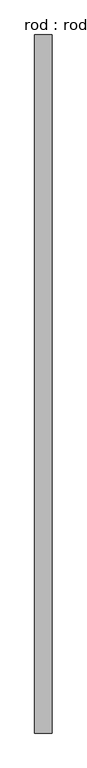
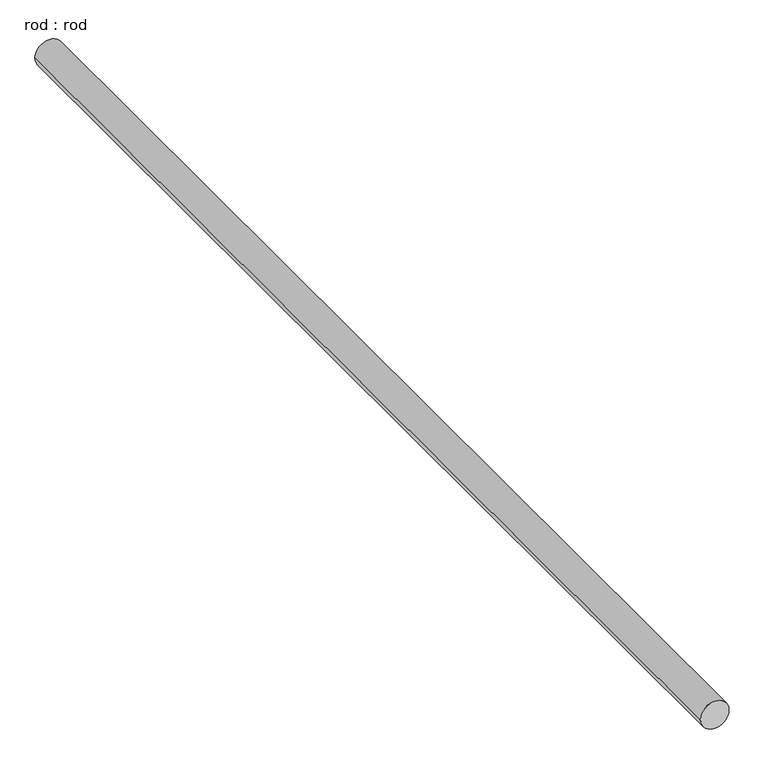
"""IFC4 building model written with IfcOpenShell, lengths in millimetres: proxy geometry, rod : rod."""

from ifc_helpers import new_model, si_unit, point, frame, frame_2d, origin, place, context, project, spatial, circle_curve, trimmed, segment, composite_curve, outline, extrude, source, transform, mapped, element, save


def rod_rod_5b3b0a5f(model_context):
    return source(origin(), model_context, "Body", "SweptSolid", [
        extrude(outline(composite_curve([segment(trimmed(circle_curve(frame_2d((0.0108462, 0.0)), 200.0), [point((0.0108462, 200.0))], [point((0.0108462, -200.0))], False, "CARTESIAN"), True, "CONTINUOUS"), segment(trimmed(circle_curve(frame_2d((0.0108462, 0.0)), 200.0), [point((0.0108462, -200.0))], [point((0.0108462, 200.0))], False, "CARTESIAN"), True, "CONTINUOUS")], self_intersect=False)), frame((0.0, -3950.3087844, 0.0), z_axis=(0.0, 1.0, 0.0), x_axis=(0.0, 0.0, 1.0)), (0.0, 0.0, 1.0), 16086.0747995),
    ])


if __name__ == "__main__":
    model = new_model("IFC4")
    model_context = context("Model", 3, world=origin())
    ifc_project = project(units=[si_unit("LENGTHUNIT", "METRE", prefix="MILLI")], contexts=[model_context])
    site = spatial("IfcSite", under=ifc_project)
    building = spatial("IfcBuilding", under=site)
    placement = place(None, origin())
    rod_rod_shape = rod_rod_5b3b0a5f(model_context)
    element("IfcBuildingElementProxy", 1, Name="rod : rod", ObjectType="rod : rod", at=placement, inside=building, context=model_context, shape_type="MappedRepresentation", body=[
        mapped(rod_rod_shape, transform((0.0, 0.0, 0.0), x_axis=(1.0, 0.0, 0.0), y_axis=(0.0, 1.0, 0.0), z_axis=(0.0, 0.0, 1.0))),
    ])
    save(model, "model.ifc")

# Revit data of these elements
# Type "rod : rod"
#   Default Elevation = 0
